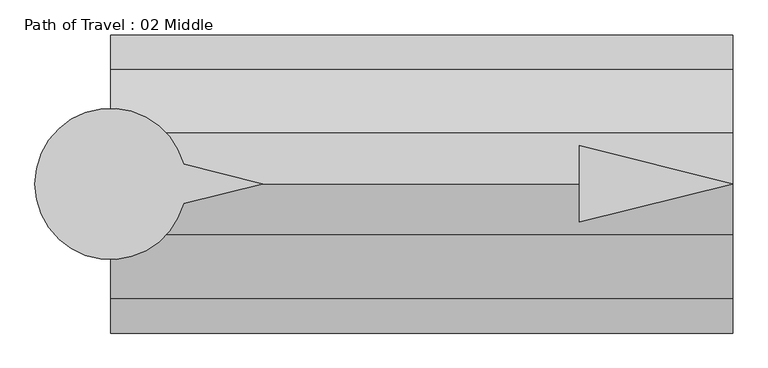
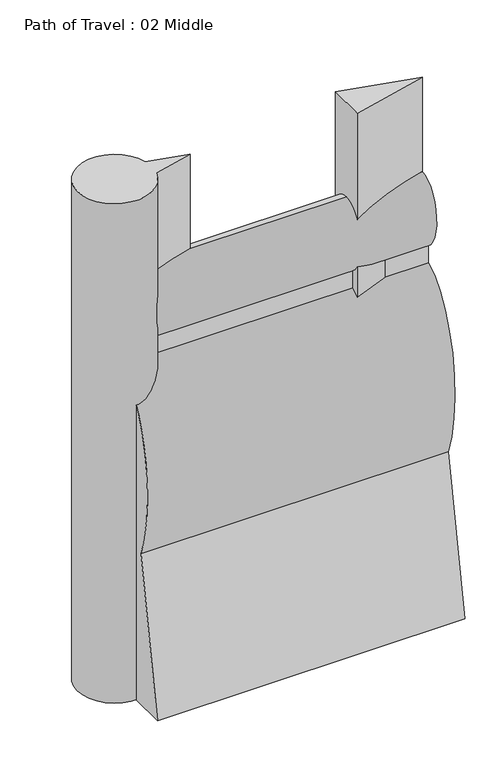
"""IFC4 building model written with IfcOpenShell, lengths in millimetres: proxy geometry, Path of Travel : 02 Middle."""

from ifc_helpers import new_model, si_unit, point, frame, frame_2d, origin, origin_with_axes, place, context, project, spatial, polyline, circle_curve, ellipse_curve, trimmed, segment, composite_curve, outline, extrude, source, transform, mapped, element, save
from ifc_brep_helpers import plane_surface, extruded_surface, advanced_brep


def path_of_travel_02_middle_a4d10025(model_context):
    return source(origin(), model_context, "Body", "SolidModel", [
        advanced_brep(
        [(227.5554837, 0.0, 1727.2), (227.5554837, 42.9018657, 1436.6534209), (227.5554837, 42.9018657, 1363.4763406), (227.5554837, 184.1186263, 643.4144547), (227.5554837, 297.5699544, 0.0), (227.5554837, 145.6574193, 0.0), (227.5554837, 0.0, 584.2), (227.5554837, -145.6574193, 0.0), (227.5554837, -297.5699544, 0.0), (227.5554837, -184.1186263, 643.4144547), (227.5554837, -42.9018657, 1363.4763406), (227.5554837, -42.9018657, 1436.6534209), (1468.4792866, 0.0, 1727.2), (1468.4792866, -42.9018657, 1436.6534209), (1468.4792866, -42.9018657, 1363.4763406), (1468.4792866, -184.1186263, 643.4144547), (1468.4792866, -297.5699544, 0.0), (1468.4792866, -145.6574193, 0.0), (1468.4792866, 0.0, 584.2), (1468.4792866, 145.6574193, 0.0), (1468.4792866, 297.5699544, 0.0), (1468.4792866, 184.1186263, 643.4144547), (1468.4792866, 42.9018657, 1363.4763406), (1468.4792866, 42.9018657, 1436.6534209)],
        [
            (0, 1, ellipse_curve(frame((227.5554837, 0.0, 1574.8), z_axis=(-1.0, 0.0, 0.0), x_axis=(0.0, 0.0, 1.0)), 152.4, 101.6)),
            (1, 2),
            (2, 3, ellipse_curve(frame((227.5554837, 0.0, 914.4), z_axis=(-1.0, 0.0, 0.0), x_axis=(0.0, 0.0, -1.0)), 457.2, 228.6)),
            (3, 4),
            (4, 5),
            (5, 6),
            (6, 7),
            (7, 8),
            (8, 9),
            (9, 10, ellipse_curve(frame((227.5554837, 0.0, 914.4), z_axis=(-1.0, 0.0, 0.0), x_axis=(0.0, 0.0, -1.0)), 457.2, 228.6)),
            (10, 11),
            (11, 0, ellipse_curve(frame((227.5554837, 0.0, 1574.8), z_axis=(-1.0, 0.0, 0.0), x_axis=(0.0, 0.0, 1.0)), 152.4, 101.6)),
            (12, 13, ellipse_curve(frame((1468.4792866, 0.0, 1574.8), z_axis=(1.0, 0.0, 0.0), x_axis=(0.0, 0.0, 1.0)), 152.4, 101.6)),
            (13, 14),
            (14, 15, ellipse_curve(frame((1468.4792866, 0.0, 914.4), z_axis=(1.0, 0.0, 0.0), x_axis=(0.0, 0.0, -1.0)), 457.2, 228.6)),
            (15, 16),
            (16, 17),
            (17, 18),
            (18, 19),
            (19, 20),
            (20, 21),
            (21, 22, ellipse_curve(frame((1468.4792866, 0.0, 914.4), z_axis=(1.0, 0.0, 0.0), x_axis=(0.0, 0.0, -1.0)), 457.2, 228.6)),
            (22, 23),
            (23, 12, ellipse_curve(frame((1468.4792866, 0.0, 1574.8), z_axis=(1.0, 0.0, 0.0), x_axis=(0.0, 0.0, 1.0)), 152.4, 101.6)),
            (0, 12),
            (23, 1),
            (22, 2),
            (21, 3),
            (20, 4),
            (19, 5),
            (18, 6),
            (17, 7),
            (16, 8),
            (15, 9),
            (14, 10),
            (13, 11),
        ],
        [
            plane_surface(frame((227.5554837, 0.0, 0.0), z_axis=(-1.0, 0.0, 0.0), x_axis=(0.0, 0.0, 1.0))),
            plane_surface(frame((1468.4792866, 0.0, 0.0), z_axis=(1.0, 0.0, 0.0), x_axis=(0.0, 0.0, 1.0))),
            extruded_surface(trimmed(ellipse_curve(frame((1468.4792866, 0.0, 1574.8), z_axis=(-1.0, 0.0, 0.0), x_axis=(0.0, 0.0, 1.0)), 152.4, 101.6), [point((1468.4792866, 0.0, 1727.2))], [point((1468.4792866, 42.9018657, 1436.6534209))], True, "CARTESIAN"), (-1240.9238029, 0.0, 0.0), 1240.9238029),
            plane_surface(frame((227.5554837, 42.9018657, 1436.6534209), z_axis=(0.0, 1.0, 0.0), x_axis=(1.0, 0.0, 0.0))),
            extruded_surface(trimmed(ellipse_curve(frame((1468.4792866, 0.0, 914.4), z_axis=(-1.0, 0.0, 0.0), x_axis=(0.0, 0.0, -1.0)), 457.2, 228.6), [point((1468.4792866, 42.9018657, 1363.4763406))], [point((1468.4792866, 184.1186263, 643.4144547))], True, "CARTESIAN"), (-1240.9238029, 0.0, 0.0), 1240.9238029),
            plane_surface(frame((227.5554837, 184.1186263, 643.4144547), z_axis=(0.0, 0.9848077530122078, 0.1736481776669322), x_axis=(1.0, 0.0, 0.0))),
            plane_surface(frame((227.5554837, 297.5699544, 0.0), z_axis=(0.0, 0.0, -1.0), x_axis=(1.0, 0.0, 0.0))),
            plane_surface(frame((227.5554837, 145.6574193, 0.0), z_axis=(0.0, -0.9702957262760199, -0.2419218955995739), x_axis=(1.0, 0.0, 0.0))),
            plane_surface(frame((227.5554837, 0.0, 584.2), z_axis=(0.0, 0.9702957262759961, -0.24192189559966923), x_axis=(1.0, 0.0, 0.0))),
            plane_surface(frame((227.5554837, -145.6574193, 0.0), z_axis=(0.0, 0.0, -1.0), x_axis=(1.0, 0.0, 0.0))),
            plane_surface(frame((227.5554837, -297.5699544, 0.0), z_axis=(0.0, -0.984807753012208, 0.17364817766693066), x_axis=(1.0, 0.0, 0.0))),
            extruded_surface(trimmed(ellipse_curve(frame((1468.4792866, 0.0, 914.4), z_axis=(-1.0, 0.0, 0.0), x_axis=(0.0, 0.0, -1.0)), 457.2, 228.6), [point((1468.4792866, -184.1186263, 643.4144547))], [point((1468.4792866, -42.9018657, 1363.4763406))], True, "CARTESIAN"), (-1240.9238029, 0.0, 0.0), 1240.9238029),
            plane_surface(frame((227.5554837, -42.9018657, 1363.4763406), z_axis=(0.0, -1.0, 0.0), x_axis=(1.0, 0.0, 0.0))),
            extruded_surface(trimmed(ellipse_curve(frame((1468.4792866, 0.0, 1574.8), z_axis=(-1.0, 0.0, 0.0), x_axis=(0.0, 0.0, 1.0)), 152.4, 101.6), [point((1468.4792866, -42.9018657, 1436.6534209))], [point((1468.4792866, 0.0, 1727.2))], True, "CARTESIAN"), (-1240.9238029, 0.0, 0.0), 1240.9238029),
        ],
        [
            (0, [[1, 2, 3, 4, 5, 6, 7, 8, 9, 10, 11, 12]]),
            (1, [[13, 14, 15, 16, 17, 18, 19, 20, 21, 22, 23, 24]]),
            (2, [[-1, 25, -24, 26]]),
            (3, [[-2, -26, -23, 27]]),
            (4, [[-3, -27, -22, 28]]),
            (5, [[-4, -28, -21, 29]]),
            (6, [[-5, -29, -20, 30]]),
            (7, [[-6, -30, -19, 31]]),
            (8, [[-7, -31, -18, 32]]),
            (9, [[-8, -32, -17, 33]]),
            (10, [[-9, -33, -16, 34]]),
            (11, [[-10, -34, -15, 35]]),
            (12, [[-11, -35, -14, 36]]),
            (13, [[-12, -36, -13, -25]]),
        ],
    ),
        extrude(outline(polyline([(1162.4741401, 76.2006338), (1468.4792866, 0.0), (1162.4741401, -76.2006338), (1162.4741401, 76.2006338)])), origin_with_axes(), (0.0, 0.0, 1.0), 2129.5973753),
        extrude(outline(composite_curve([segment(polyline([(372.7837828, 39.4440225), (531.182385, 0.0), (372.7837828, -39.4440225)]), True, "CONTINUOUS"), segment(trimmed(circle_curve(frame_2d((227.2200886, 0.0)), 150.8131956), [point((372.7837828, -39.4440225))], [point((372.7837828, 39.4440225))], False, "CARTESIAN"), True, "CONTINUOUS")], self_intersect=False)), origin_with_axes(), (0.0, 0.0, 1.0), 2129.5973753),
    ])


if __name__ == "__main__":
    model = new_model("IFC4")
    model_context = context("Model", 3, world=origin())
    ifc_project = project(units=[si_unit("LENGTHUNIT", "METRE", prefix="MILLI")], contexts=[model_context])
    site = spatial("IfcSite", under=ifc_project)
    building = spatial("IfcBuilding", under=site)
    placement = place(None, origin())
    path_of_travel_02_middle_shape = path_of_travel_02_middle_a4d10025(model_context)
    element("IfcBuildingElementProxy", 1, Name="Path of Travel : 02 Middle", ObjectType="Path of Travel : 02 Middle", at=placement, inside=building, context=model_context, shape_type="MappedRepresentation", body=[
        mapped(path_of_travel_02_middle_shape, transform((0.0, 0.0, 0.0), x_axis=(1.0, 0.0, 0.0), y_axis=(0.0, 1.0, 0.0), z_axis=(0.0, 0.0, 1.0))),
    ])
    save(model, "model.ifc")

# Revit data of these elements
# Type "Path of Travel : 02 Middle"
#   Path of Egress [instance default] = 4' - 0"
#   built-in parameter 1001306 [instance default] = 4 (stored number, unit not read)
#   Dot at Start = no
#   Arrow in Middle = yes
#   Arrow at End = no
#   Egress Path = none
# Element 1 (IfcBuildingElementProxy, "Path of Travel : 02 Middle")
#   Path of Egress = 4' - 0.85527"
#   built-in parameter 1001306 = 4.07127 (stored number, unit not read)
#   Materials on its faces: "Egress Path Solid", "solid"
# Materials
#   "Egress Path Solid": class "Unassigned", colour RGB 255 128 64, transparency 0.75, Comments = "Rendering appearance not upgraded "
#   "solid": class "Generic", colour RGB 120 120 120, transparency 0, Cost = 0
